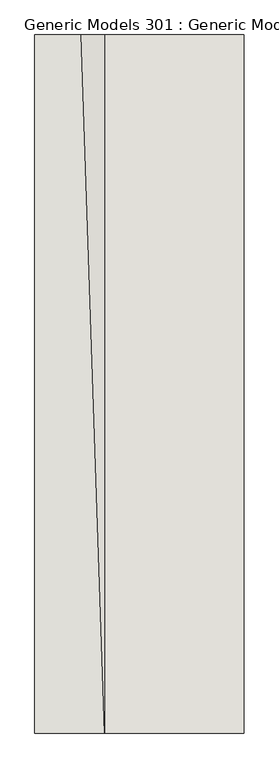
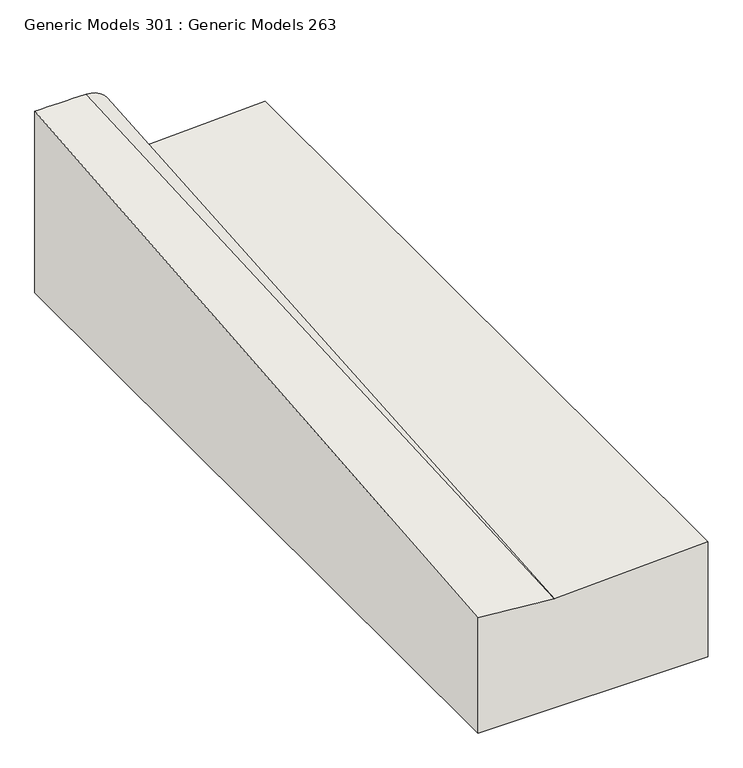
"""IFC4 building model written with IfcOpenShell, lengths in millimetres: wall geometry, Generic Models 301 : Generic Models 263."""

from ifc_helpers import new_model, si_unit, frame, origin, place, context, project, spatial, circle_curve, source, transform, mapped, element, save
from ifc_brep_helpers import plane_surface, spline_surface, advanced_brep


def generic_models_301_generic_models_263_c6164b38(model_context):
    return source(origin(), model_context, "Body", "AdvancedBrep", [
        advanced_brep(
        [(91579.9797726, 582.5727422, -139.1379392), (91579.9797726, 582.5727422, -381.0), (92037.1797726, 582.5727422, -381.0), (92037.1797726, 582.5727422, -139.7), (91732.3797726, 582.5727422, -152.4), (91579.9797726, 2106.5727422, 0.0), (91681.5797726, 2106.5727422, 0.0), (91732.3797726, 2106.5727422, -50.8), (91732.3797726, 2106.5727422, -152.4), (92037.1797726, 2106.5727422, -139.7), (92037.1797726, 2106.5727422, -381.0), (91579.9797726, 2106.5727422, -381.0)],
        [
            (0, 1),
            (1, 2),
            (2, 3),
            (3, 4),
            (4, 0),
            (5, 6),
            (6, 7, circle_curve(frame((91681.5797726, 2106.5727422, -50.8), z_axis=(0.0, 1.0, 0.0), x_axis=(1.0, 0.0, 0.0)), 50.8)),
            (7, 8),
            (8, 9),
            (9, 10),
            (10, 11),
            (11, 5),
            (11, 1),
            (0, 5),
            (10, 2),
            (9, 3),
            (7, 4),
            (4, 8),
            (6, 4),
        ],
        [
            plane_surface(frame((91793.3397726, 582.5727422, -238.6475878), z_axis=(0.0, -1.0, 0.0), x_axis=(1.0, 0.0, 0.0))),
            plane_surface(frame((91768.6654869, 2106.5727422, -157.8428571), z_axis=(0.0, 1.0, 0.0), x_axis=(1.0, 0.0, 0.0))),
            plane_surface(frame((91579.9797726, 2106.5727422, -190.5), z_axis=(-1.0, 0.0, 0.0), x_axis=(0.0, 0.0, -1.0))),
            plane_surface(frame((91808.5797726, 2106.5727422, -381.0), z_axis=(0.0, 0.0, -1.0), x_axis=(1.0, 0.0, 0.0))),
            plane_surface(frame((92037.1797726, 2106.5727422, -260.35), z_axis=(1.0, 0.0, 0.0), x_axis=(0.0, 0.0, 1.0))),
            plane_surface(frame((91732.3797726, 2106.5727422, -101.6), z_axis=(1.0, 0.0, 0.0), x_axis=(0.0, 0.0, 1.0))),
            spline_surface(2, 1, [[(91732.3797726, 2106.5727422, -50.8), (91732.3797726, 582.5727422, -152.4)], [(91732.3797726, 2106.5727422, 2.9132252166164108e-12), (91732.3797726, 582.5727422, -152.4)], [(91681.5797726, 2106.5727422, 0.0), (91732.3797726, 582.5727422, -152.4)]], [3, 3], [2, 2], [0.0, 1.0], [0.0, 1.0], weights=[[1.0, 1.0], [0.7071067811865273, 0.7071067811865273], [1.0, 1.0]]),
            spline_surface(1, 1, [[(91681.5797726, 2106.5727422, 0.0), (91732.3797726, 582.5727422, -152.4)], [(91579.9797726, 2106.5727422, 0.0), (91579.9797726, 582.5727422, -139.1379392)]], [2, 2], [2, 2], [0.0, 1.0], [0.0, 1.0]),
            plane_surface(frame((91884.7797726, 2106.5727422, -146.05), z_axis=(-0.04163054471218724, 0.0, 0.9991330730923517), x_axis=(-0.9991330730923517, 0.0, -0.04163054471218724))),
        ],
        [
            (0, [[1, 2, 3, 4, 5]]),
            (1, [[6, 7, 8, 9, 10, 11, 12]]),
            (2, [[-12, 13, -1, 14]]),
            (3, [[-11, 15, -2, -13]]),
            (4, [[-10, 16, -3, -15]]),
            (5, [[-8, 17, 18]]),
            (6, [[-7, 19, -17]]),
            (7, [[-6, -14, -5, -19]]),
            (8, [[-9, -18, -4, -16]]),
        ],
    ),
    ])


if __name__ == "__main__":
    model = new_model("IFC4")
    model_context = context("Model", 3, world=origin())
    ifc_project = project(units=[si_unit("LENGTHUNIT", "METRE", prefix="MILLI")], contexts=[model_context])
    site = spatial("IfcSite", under=ifc_project)
    building = spatial("IfcBuilding", under=site)
    placement = place(None, origin())
    generic_models_301_generic_models_263_shape = generic_models_301_generic_models_263_c6164b38(model_context)
    element("IfcWall", 1, ObjectType="Generic Models 301 : Generic Models 263", at=placement, inside=building, context=model_context, shape_type="MappedRepresentation", body=[
        mapped(generic_models_301_generic_models_263_shape, transform((0.0, 0.0, 0.0), x_axis=(1.0, 0.0, 0.0), y_axis=(0.0, 1.0, 0.0), z_axis=(0.0, 0.0, 1.0))),
    ])
    save(model, "model.ifc")

# Revit data of these elements
# Element 1 (IfcWall, "Generic Models 301 : Generic Models 263")
#   Materials on its faces: "CONCRETE CURB"
# Materials
#   "CONCRETE CURB": class "Concrete", colour RGB 191 191 191, transparency 0, Description = "Cast-in-place concrete", Cost = 0
